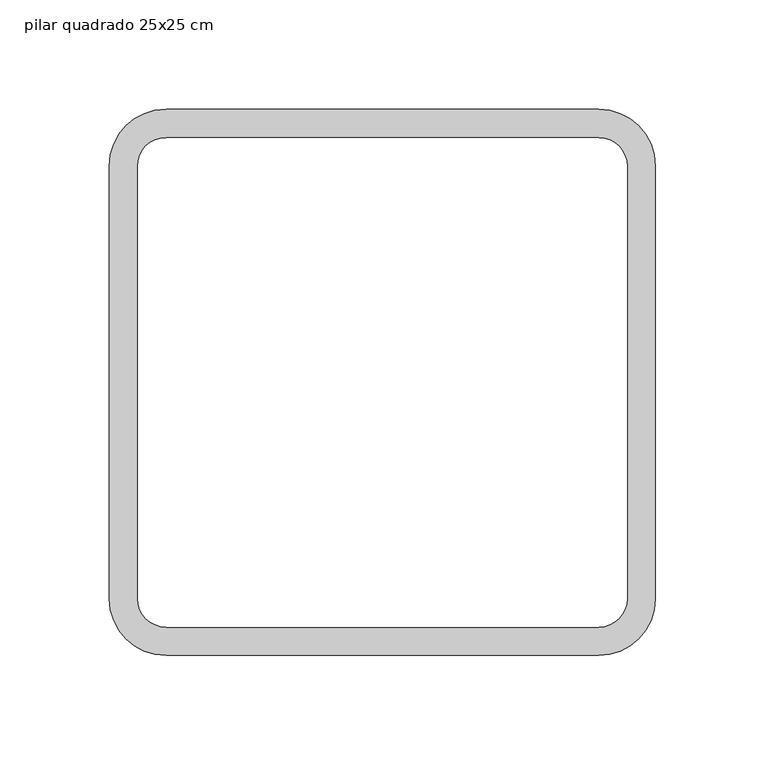
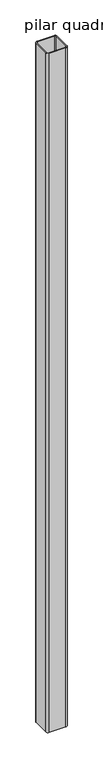
"""IFC4 building model written with IfcOpenShell, lengths in millimetres: column geometry, CEV-Corte da estrutura vazado-Coluna : pilar quadrado 25x25 cm."""

import ifcopenshell
import ifcopenshell.guid

model = None  # the IFC model being written
_history = None  # IfcOwnerHistory: only IFC2X3 demands one
_inside = {}  # id of a spatial element -> (the spatial element, [elements in it])
_under = {}  # id of a project, library or spatial element -> (it, [spatial elements below it])
_declared = {}  # id of a project -> (the project, [libraries it declares])
_typed = {}  # id of a type object -> (the type object, [elements of that type])
_made_of = {}  # id of a material, layer set ... -> (it, [elements and type objects made of it])


def new_model(schema):
    """Start an empty IFC model of exactly this schema.

    Asked for "IFC4X3", IfcOpenShell would pick the latest addendum, in which some entities
    have other attributes; the version numbers below select the first issue.
    IFC2X3 requires an IfcOwnerHistory on every rooted entity: one is made here for all.
    """
    global model, _history
    if schema == "IFC4X3":
        model = ifcopenshell.file(schema_version=(4, 3, 0, 0))
    else:
        model = ifcopenshell.file(schema=schema)
    _inside.clear()
    _under.clear()
    _declared.clear()
    _typed.clear()
    _made_of.clear()
    _history = None
    if model.schema == "IFC2X3":
        org = make("IfcOrganization", Name="unknown")
        user = make(
            "IfcPersonAndOrganization",
            ThePerson=make("IfcPerson", FamilyName="unknown"),
            TheOrganization=org,
        )
        app = make(
            "IfcApplication",
            ApplicationDeveloper=org,
            Version="unknown",
            ApplicationFullName="unknown",
            ApplicationIdentifier="unknown",
        )
        _history = make(
            "IfcOwnerHistory",
            OwningUser=user,
            OwningApplication=app,
            ChangeAction="ADDED",
            CreationDate=0,
        )
    return model


def make(cls, **values):
    """One entity of the class cls with the attributes given. An attribute that is None is left unset."""
    return model.create_entity(
        cls, **{name: value for name, value in values.items() if value is not None}
    )


def rooted(cls, **values):
    """An entity with a GlobalId (a new one), such as an element, a storey or a relation."""
    return make(cls, GlobalId=ifcopenshell.guid.new(), OwnerHistory=_history, **values)


def si_unit(unit_type, name, prefix=None):
    """IfcSIUnit, for example si_unit("LENGTHUNIT", "METRE", prefix="MILLI")."""
    return make("IfcSIUnit", UnitType=unit_type, Prefix=prefix, Name=name)


def assignment(units):
    """IfcUnitAssignment: the units of a project."""
    return None if units is None else make("IfcUnitAssignment", Units=units)


def point(xyz):
    """IfcCartesianPoint."""
    return None if xyz is None else make("IfcCartesianPoint", Coordinates=xyz)


def direction(xyz):
    """IfcDirection."""
    return None if xyz is None else make("IfcDirection", DirectionRatios=xyz)


def frame(location, z_axis=None, x_axis=None):
    """IfcAxis2Placement3D, a coordinate frame: its origin and axes. An axis left out is left unset."""
    return make(
        "IfcAxis2Placement3D",
        Location=point(location),
        Axis=direction(z_axis),
        RefDirection=direction(x_axis),
    )


def frame_2d(location, x_axis=None):
    """IfcAxis2Placement2D, a coordinate frame in the plane: its origin and x axis."""
    return make(
        "IfcAxis2Placement2D", Location=point(location), RefDirection=direction(x_axis)
    )


def origin():
    """The frame at (0, 0, 0) with its axes left unset."""
    return frame((0.0, 0.0, 0.0))


def place(relative_to, where):
    """IfcLocalPlacement: puts the frame where relative to a parent placement (None: the world)."""
    return make(
        "IfcLocalPlacement", PlacementRelTo=relative_to, RelativePlacement=where
    )


def context(
    kind, dimensions, precision=None, world=None, true_north=None, identifier=None
):
    """IfcGeometricRepresentationContext, for example the 3D "Model" context."""
    return make(
        "IfcGeometricRepresentationContext",
        ContextIdentifier=identifier,
        ContextType=kind,
        CoordinateSpaceDimension=dimensions,
        Precision=precision,
        WorldCoordinateSystem=world,
        TrueNorth=true_north,
    )


def project(units=None, contexts=None):
    """IfcProject with its units and contexts."""
    return rooted(
        "IfcProject",
        Name="project",
        RepresentationContexts=contexts,
        UnitsInContext=assignment(units),
    )


def spatial(cls, under=None, at=None, **own):
    """A site, building, storey or space (cls), placed at a placement, below another one or the project."""
    s = rooted(cls, ObjectPlacement=at, **own)
    if under is not None:
        _under.setdefault(under.id(), (under, []))[1].append(s)
    return s


def polyline(points):
    """IfcPolyline through the points."""
    return make("IfcPolyline", Points=[point(p) for p in points])


def circle_curve(where, radius):
    """IfcCircle in the frame where."""
    return make("IfcCircle", Position=where, Radius=radius)


def trimmed(basis, trim1, trim2, sense, master):
    """IfcTrimmedCurve: the piece of a basis curve between two trims."""
    return make(
        "IfcTrimmedCurve",
        BasisCurve=basis,
        Trim1=trim1,
        Trim2=trim2,
        SenseAgreement=sense,
        MasterRepresentation=master,
    )


def segment(curve, same_sense, transition):
    """IfcCompositeCurveSegment."""
    return make(
        "IfcCompositeCurveSegment",
        Transition=transition,
        SameSense=same_sense,
        ParentCurve=curve,
    )


def composite_curve(segments, self_intersect=None):
    """IfcCompositeCurve: segments joined end to end."""
    return make("IfcCompositeCurve", Segments=segments, SelfIntersect=self_intersect)


def outline(outer, holes=None, kind="AREA"):
    """IfcArbitraryClosedProfileDef: a profile drawn as a closed curve; with holes, ...WithVoids."""
    if holes is None:
        return make("IfcArbitraryClosedProfileDef", ProfileType=kind, OuterCurve=outer)
    return make(
        "IfcArbitraryProfileDefWithVoids",
        ProfileType=kind,
        OuterCurve=outer,
        InnerCurves=holes,
    )


def extrude(swept, where, along, depth):
    """IfcExtrudedAreaSolid: the profile swept, set in the frame where, extruded along a direction by depth."""
    return make(
        "IfcExtrudedAreaSolid",
        SweptArea=swept,
        Position=where,
        ExtrudedDirection=direction(along),
        Depth=depth,
    )


def shape(context_of_items, identifier, shape_type, items):
    """IfcShapeRepresentation: the items that make up one representation, for example the "Body"."""
    return make(
        "IfcShapeRepresentation",
        ContextOfItems=context_of_items,
        RepresentationIdentifier=identifier,
        RepresentationType=shape_type,
        Items=items,
    )


def source(mapping_origin, context_of_items, identifier, shape_type, items):
    """IfcRepresentationMap: a shape defined once, which mapped items show again and again."""
    return make(
        "IfcRepresentationMap",
        MappingOrigin=mapping_origin,
        MappedRepresentation=shape(context_of_items, identifier, shape_type, items),
    )


def transform(
    local_origin,
    x_axis=None,
    y_axis=None,
    z_axis=None,
    scale=None,
    scale2=None,
    scale3=None,
    uniform=True,
):
    """IfcCartesianTransformationOperator3D, or its non-uniform kind. x_axis, y_axis, z_axis: its Axis1, 2, 3."""
    if uniform:
        return make(
            "IfcCartesianTransformationOperator3D",
            Axis1=direction(x_axis),
            Axis2=direction(y_axis),
            LocalOrigin=point(local_origin),
            Scale=scale,
            Axis3=direction(z_axis),
        )
    return make(
        "IfcCartesianTransformationOperator3DnonUniform",
        Axis1=direction(x_axis),
        Axis2=direction(y_axis),
        LocalOrigin=point(local_origin),
        Scale=scale,
        Axis3=direction(z_axis),
        Scale2=scale2,
        Scale3=scale3,
    )


def mapped(mapping_source, mapping_target):
    """IfcMappedItem: shows the shape of a source again, moved by a transform."""
    return make(
        "IfcMappedItem", MappingSource=mapping_source, MappingTarget=mapping_target
    )


def made_of(thing, what):
    """Note that an element or type object is made of a material, layer set ...; save() writes the relation."""
    if what is not None:
        _made_of.setdefault(what.id(), (what, []))[1].append(thing)
    return thing


def element(
    cls,
    number,
    at=None,
    inside=None,
    cuts=None,
    type_object=None,
    material=None,
    context=None,
    identifier="Body",
    shape_type=None,
    held_by="IfcProductDefinitionShape",
    body=None,
    shapes=None,
    **own,
):
    """One element of the class cls, such as IfcWall. Its Tag is "e" and its number.

    at: its placement. inside: the storey or other place that contains it. cuts: it is an
    opening in that element (IfcRelVoidsElement). A single representation is given by context,
    identifier, shape_type and body (its items); several are given by shapes. held_by: the class
    of the entity that holds the representations. save() writes the other relations.
    """
    e = rooted(cls, Tag="e%d" % number, ObjectPlacement=at, **own)
    if body is not None:
        shapes = [shape(context, identifier, shape_type, body)]
    if shapes is not None:
        e.Representation = make(held_by, Representations=shapes)
    if inside is not None:
        _inside.setdefault(inside.id(), (inside, []))[1].append(e)
    if cuts is not None:
        rooted(
            "IfcRelVoidsElement", RelatingBuildingElement=cuts, RelatedOpeningElement=e
        )
    if type_object is not None:
        _typed.setdefault(type_object.id(), (type_object, []))[1].append(e)
    return made_of(e, material)


def aggregate(whole, parts):
    """IfcRelAggregates: a whole, such as a stair, and the parts it consists of."""
    return rooted("IfcRelAggregates", RelatingObject=whole, RelatedObjects=parts)


def save(model, path):
    """Write the relations noted so far, then the file.

    IfcRelAggregates (storeys below a building ...), IfcRelContainedInSpatialStructure (elements
    in a storey), IfcRelDefinesByType, IfcRelAssociatesMaterial and IfcRelDeclares: one each for
    every whole, place, type object, material and project.
    """
    for whole, parts in _under.values():
        aggregate(whole, parts)
    for where, things in _inside.values():
        rooted(
            "IfcRelContainedInSpatialStructure",
            RelatedElements=things,
            RelatingStructure=where,
        )
    for kind, things in _typed.values():
        rooted("IfcRelDefinesByType", RelatedObjects=things, RelatingType=kind)
    for what, things in _made_of.values():
        rooted("IfcRelAssociatesMaterial", RelatedObjects=things, RelatingMaterial=what)
    for by, libraries in _declared.values():
        rooted("IfcRelDeclares", RelatingContext=by, RelatedDefinitions=libraries)
    model.write(path)


def pilar_quadrado_25x25_cm_e96a00db(model_context):
    return source(origin(), model_context, "Body", "SweptSolid", [
        extrude(outline(composite_curve([segment(trimmed(circle_curve(frame_2d((99.0, 99.0)), 26.0), [point((99.0, 125.0))], [point((125.0, 99.0))], False, "CARTESIAN"), True, "CONTINUOUS"), segment(polyline([(125.0, 99.0), (125.0, -99.0)]), True, "CONTINUOUS"), segment(trimmed(circle_curve(frame_2d((99.0, -99.0)), 26.0), [point((125.0, -99.0))], [point((99.0, -125.0))], False, "CARTESIAN"), True, "CONTINUOUS"), segment(polyline([(99.0, -125.0), (-99.0, -125.0)]), True, "CONTINUOUS"), segment(trimmed(circle_curve(frame_2d((-99.0, -99.0)), 26.0), [point((-99.0, -125.0))], [point((-125.0, -99.0))], False, "CARTESIAN"), True, "CONTINUOUS"), segment(polyline([(-125.0, -99.0), (-125.0, 99.0)]), True, "CONTINUOUS"), segment(trimmed(circle_curve(frame_2d((-99.0, 99.0)), 26.0), [point((-125.0, 99.0))], [point((-99.0, 125.0))], False, "CARTESIAN"), True, "CONTINUOUS"), segment(polyline([(-99.0, 125.0), (99.0, 125.0)]), True, "CONTINUOUS")], self_intersect=False), holes=[composite_curve([segment(polyline([(99.0, 112.0), (-99.0, 112.0)]), True, "CONTINUOUS"), segment(trimmed(circle_curve(frame_2d((-99.0, 99.0)), 13.0), [point((-99.0, 112.0))], [point((-112.0, 99.0))], True, "CARTESIAN"), True, "CONTINUOUS"), segment(polyline([(-112.0, 99.0), (-112.0, -99.0)]), True, "CONTINUOUS"), segment(trimmed(circle_curve(frame_2d((-99.0, -99.0)), 13.0), [point((-112.0, -99.0))], [point((-99.0, -112.0))], True, "CARTESIAN"), True, "CONTINUOUS"), segment(polyline([(-99.0, -112.0), (99.0, -112.0)]), True, "CONTINUOUS"), segment(trimmed(circle_curve(frame_2d((99.0, -99.0)), 13.0), [point((99.0, -112.0))], [point((112.0, -99.0))], True, "CARTESIAN"), True, "CONTINUOUS"), segment(polyline([(112.0, -99.0), (112.0, 99.0)]), True, "CONTINUOUS"), segment(trimmed(circle_curve(frame_2d((99.0, 99.0)), 13.0), [point((112.0, 99.0))], [point((99.0, 112.0))], True, "CARTESIAN"), True, "CONTINUOUS")], self_intersect=False)]), frame((0.0, 0.0, 39630.0), z_axis=(0.0, 0.0, 1.0), x_axis=(1.0, 0.0, 0.0)), (0.0, 0.0, 1.0), 8535.0),
    ])


if __name__ == "__main__":
    model = new_model("IFC4")
    model_context = context("Model", 3, world=origin())
    ifc_project = project(units=[si_unit("LENGTHUNIT", "METRE", prefix="MILLI")], contexts=[model_context])
    site = spatial("IfcSite", under=ifc_project)
    building = spatial("IfcBuilding", under=site)
    placement = place(None, origin())
    pilar_quadrado_25x25_cm_shape = pilar_quadrado_25x25_cm_e96a00db(model_context)
    element("IfcColumn", 1, ObjectType="CEV-Corte da estrutura vazado-Coluna : pilar quadrado 25x25 cm", at=placement, inside=building, context=model_context, shape_type="MappedRepresentation", body=[
        mapped(pilar_quadrado_25x25_cm_shape, transform((0.0, 0.0, 0.0), x_axis=(1.0, 0.0, 0.0), y_axis=(0.0, 1.0, 0.0), z_axis=(0.0, 0.0, 1.0))),
    ])
    save(model, "model.ifc")

# Revit data of these elements
# Type "CEV-Corte da estrutura vazado-Coluna : pilar quadrado 25x25 cm"
#   Forma = "Quadrado"
#   W = 0.0258
#   Ht = 0.25 m
#   b = 0.25 m
#   kr = 0.026 m
#   t = 0.013 m
#   A = 0.000317 m²
#   Structural Material [instance default] = Aço, 45-345
#   Assembly Code = ""
# Element 1 (IfcColumn, "CEV-Corte da estrutura vazado-Coluna : pilar quadrado 25x25 cm")
#   Materials on its faces: "Aço, 45-345"
# Materials
#   "Aço, 45-345": class "Metal", colour RGB 247 247 247, transparency 0, Description = "Aço 345 MPa", Cost = 0
